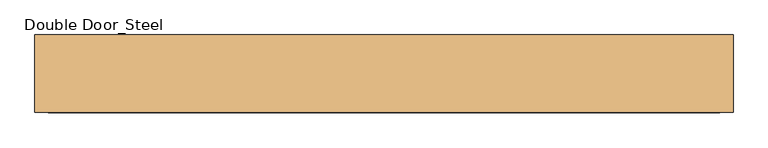
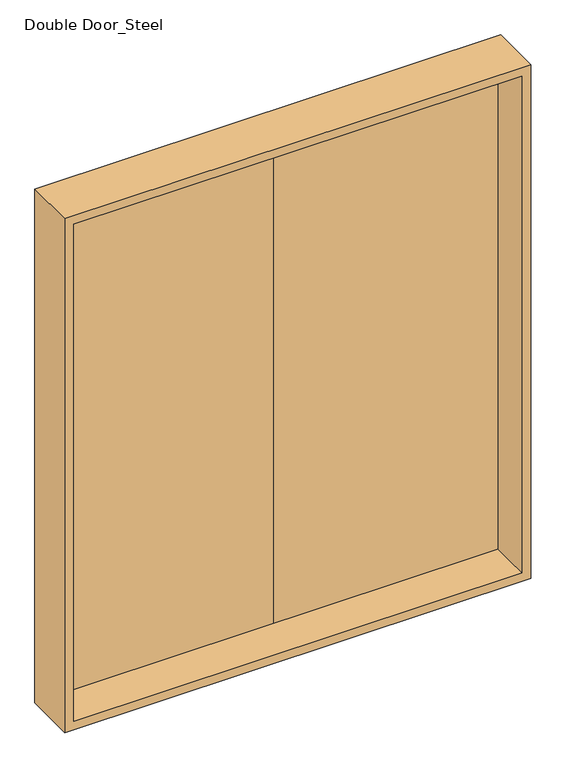
"""IFC4 building model written with IfcOpenShell, lengths in millimetres: door geometry, Double Door_Steel : H_DR_AR_B12_Double Door_Steel_W2000xH2100."""

from ifc_helpers import new_model, si_unit, frame, origin, place, context, project, spatial, polyline, outline, extrude, faceted_brep, source, transform, mapped, element, save


def double_door_steel_22a565f0(model_context):
    return source(origin(), model_context, "Body", "SolidModel", [
        extrude(outline(polyline([(880.0, 60.0), (0.0, 60.0), (0.0, 100.0), (880.0, 100.0), (880.0, 60.0)])), frame((0.0, 0.0, 20.0), z_axis=(0.0, 0.0, 1.0), x_axis=(1.0, 0.0, 0.0)), (0.0, 0.0, 1.0), 2060.0),
        extrude(outline(polyline([(0.0, 60.0), (-880.0, 60.0), (-880.0, 100.0), (0.0, 100.0), (0.0, 60.0)])), frame((0.0, 0.0, 20.0), z_axis=(0.0, 0.0, 1.0), x_axis=(1.0, 0.0, 0.0)), (0.0, 0.0, 1.0), 2060.0),
        faceted_brep([(900.0, -100.0, 2100.0), (900.0, 100.0, 2100.0), (-900.0, 100.0, 2100.0), (-900.0, -100.0, 2100.0), (865.0, 60.0, 2065.0), (865.0, -100.0, 2065.0), (-865.0, -100.0, 2065.0), (-865.0, 60.0, 2065.0), (880.0, 100.0, 2080.0), (880.0, 60.0, 2080.0), (-880.0, 60.0, 2080.0), (-880.0, 100.0, 2080.0), (-900.0, 100.0, 0.0), (-900.0, -100.0, 0.0), (-865.0, -100.0, 35.0), (-865.0, 60.0, 35.0), (-880.0, 60.0, 20.0), (-880.0, 100.0, 20.0), (900.0, 100.0, 0.0), (880.0, 100.0, 20.0), (900.0, -100.0, 0.0), (865.0, -100.0, 35.0), (865.0, 60.0, 35.0), (880.0, 60.0, 20.0)], [[[0, 1, 2, 3]], [[4, 5, 6, 7]], [[8, 9, 10, 11]], [[3, 2, 12, 13]], [[7, 6, 14, 15]], [[11, 10, 16, 17]], [[18, 12, 2, 1], [8, 11, 17, 19]], [[13, 12, 18, 20]], [[0, 3, 13, 20], [21, 14, 6, 5]], [[15, 14, 21, 22]], [[23, 16, 10, 9], [4, 7, 15, 22]], [[17, 16, 23, 19]], [[20, 18, 1, 0]], [[22, 21, 5, 4]], [[19, 23, 9, 8]]]),
    ])


if __name__ == "__main__":
    model = new_model("IFC4")
    model_context = context("Model", 3, world=origin())
    ifc_project = project(units=[si_unit("LENGTHUNIT", "METRE", prefix="MILLI")], contexts=[model_context])
    site = spatial("IfcSite", under=ifc_project)
    building = spatial("IfcBuilding", under=site)
    placement = place(None, origin())
    double_door_steel_shape = double_door_steel_22a565f0(model_context)
    element("IfcDoor", 1, ObjectType="Double Door_Steel : H_DR_AR_B12_Double Door_Steel_W2000xH2100", at=placement, inside=building, context=model_context, shape_type="MappedRepresentation", body=[
        mapped(double_door_steel_shape, transform((0.0, 0.0, 0.0), x_axis=(1.0, 0.0, 0.0), y_axis=(0.0, 1.0, 0.0), z_axis=(0.0, 0.0, 1.0))),
    ])
    save(model, "model.ifc")

# Revit data of these elements
# Type "Double Door_Steel : H_DR_AR_B12_Double Door_Steel_W2000xH2100"
#   Type Mark = ""
#   프레임 = ""
#   철물 = ""
#   유리/마감 = ""
#   위치/개소 = ""
#   부호 = "1/SD"
#   문번호 = ""
#   문기호 = "SD"
#   Analytic Construction = "<None>"
#   Height = 2100 mm
#   Width = 1800 mm
#   Define Thermal Properties by = 1
#   문 틀 = none
#   문 = none
#   Function = (empty or 0)
#   Assembly Code = ""
#   Wall Closure = (empty or 0)
